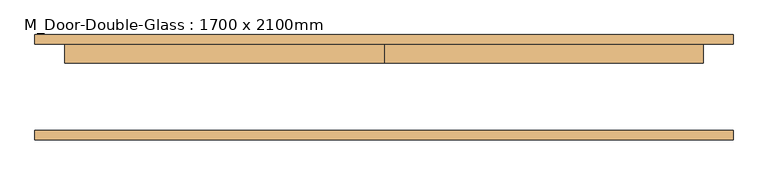
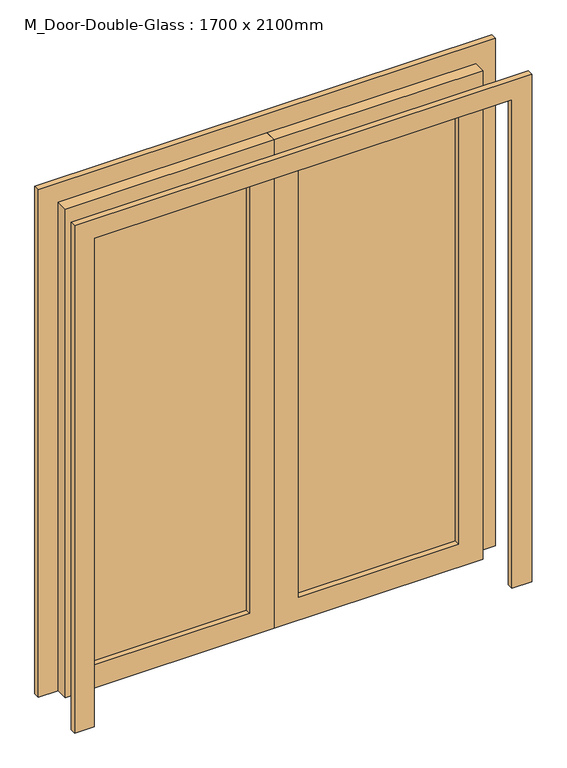
"""IFC4 building model written with IfcOpenShell, lengths in millimetres: door geometry, M_Door-Double-Glass : 1700 x 2100mm."""

from ifc_helpers import new_model, si_unit, frame, origin, place, context, project, spatial, polyline, outline, extrude, source, transform, mapped, element, save


def m_door_double_glass_1700_x_2100mm_d150df18(model_context):
    return source(origin(), model_context, "Body", "SweptSolid", [
        extrude(outline(polyline([(2100.0, -850.0), (0.0, -850.0), (0.0, 0.0), (2100.0, 0.0), (2100.0, -850.0)]), holes=[polyline([(2000.0, -750.0), (2000.0, -100.0), (100.0, -100.0), (100.0, -750.0), (2000.0, -750.0)])]), frame((0.0, 67.38125, 0.0), z_axis=(0.0, 1.0, 0.0), x_axis=(0.0, 0.0, 1.0)), (0.0, 0.0, 1.0), 50.0),
        extrude(outline(polyline([(2100.0, 850.0), (2100.0, 0.0), (0.0, 0.0), (0.0, 850.0), (2100.0, 850.0)]), holes=[polyline([(2000.0, 750.0), (100.0, 750.0), (100.0, 100.0), (2000.0, 100.0), (2000.0, 750.0)])]), frame((0.0, 67.38125, 0.0), z_axis=(0.0, 1.0, 0.0), x_axis=(0.0, 0.0, 1.0)), (0.0, 0.0, 1.0), 50.0),
        extrude(outline(polyline([(100.0, 95.55625), (750.0, 95.55625), (750.0, 89.20625), (100.0, 89.20625), (100.0, 95.55625)])), frame((0.0, 0.0, 100.0), z_axis=(0.0, 0.0, 1.0), x_axis=(1.0, 0.0, 0.0)), (0.0, 0.0, 1.0), 1900.0),
        extrude(outline(polyline([(-750.0, 95.55625), (-100.0, 95.55625), (-100.0, 89.20625), (-750.0, 89.20625), (-750.0, 95.55625)])), frame((0.0, 0.0, 100.0), z_axis=(0.0, 0.0, 1.0), x_axis=(1.0, 0.0, 0.0)), (0.0, 0.0, 1.0), 1900.0),
        extrude(outline(polyline([(0.0, 930.0), (2180.0, 930.0), (2180.0, -930.0), (0.0, -930.0), (0.0, -850.0), (2100.0, -850.0), (2100.0, 850.0), (0.0, 850.0), (0.0, 930.0)])), frame((0.0, 117.38125, 0.0), z_axis=(0.0, 1.0, 0.0), x_axis=(0.0, 0.0, 1.0)), (0.0, 0.0, 1.0), 25.0),
        extrude(outline(polyline([(0.0, 930.0), (2180.0, 930.0), (2180.0, -930.0), (0.0, -930.0), (0.0, -850.0), (2100.0, -850.0), (2100.0, 850.0), (0.0, 850.0), (0.0, 930.0)])), frame((0.0, -137.61875, 0.0), z_axis=(0.0, 1.0, 0.0), x_axis=(0.0, 0.0, 1.0)), (0.0, 0.0, 1.0), 25.0),
    ])


if __name__ == "__main__":
    model = new_model("IFC4")
    model_context = context("Model", 3, world=origin())
    ifc_project = project(units=[si_unit("LENGTHUNIT", "METRE", prefix="MILLI")], contexts=[model_context])
    site = spatial("IfcSite", under=ifc_project)
    building = spatial("IfcBuilding", under=site)
    placement = place(None, origin())
    m_door_double_glass_1700_x_2100mm_shape = m_door_double_glass_1700_x_2100mm_d150df18(model_context)
    element("IfcDoor", 1, ObjectType="M_Door-Double-Glass : 1700 x 2100mm", at=placement, inside=building, context=model_context, shape_type="MappedRepresentation", body=[
        mapped(m_door_double_glass_1700_x_2100mm_shape, transform((0.0, 0.0, 0.0), x_axis=(1.0, 0.0, 0.0), y_axis=(0.0, 1.0, 0.0), z_axis=(0.0, 0.0, 1.0))),
    ])
    save(model, "model.ifc")

# Revit data of these elements
# Type "M_Door-Double-Glass : 1700 x 2100mm"
#   Type Mark = "42"
#   Construction Type Id = "opn-d45"
#   Assembly Code = "C1020"
#   Analytic Construction = "Wood frame, double glass door "
#   W = 85 cm
#   Thickness = 5 cm
#   Thermal Resistance (R) = 0.31964 (m²·K)/W
#   Swing Angle [instance default] = 90.00°
#   Heat Transfer Coefficient (U) = 3.12872 W/(m²·K)
#   Height = 210 cm
#   Bottom Rail = 10 cm
#   Top Rail = 10 cm
#   Stiles = 10 cm
#   Trim Projection = 2.5 cm
#   Trim Width = 8 cm
#   Width = 170 cm
#   Glazing = Glass
#   Panel Material = Wood - Birch - Solid Stained Light Low Gloss
#   Trim Material = Paint - Sienna
#   Visual Light Transmittance = 0
#   Solar Heat Gain Coefficient = 0
#   Function = (empty or 0)
#   Wall Closure = (empty or 0)
# Element 1 (IfcDoor, "M_Door-Double-Glass : 1700 x 2100mm")
#   Materials on its faces: "Wood - Birch - Solid Stained Light Low Gloss", "Paint - Sienna", "Glass"
# Materials
#   "Glass": class "Glass", colour RGB 0 128 192, transparency 0.9, Description = "Soda Lime Glass", Cost = 0
#   "Wood - Birch - Solid Stained Light Low Gloss": class "Wood", colour RGB 210 159 95, transparency 0, Cost = 0
#   "Paint - Sienna": class "Miscellaneous", colour RGB 118 70 51, transparency 0, Cost = 0
